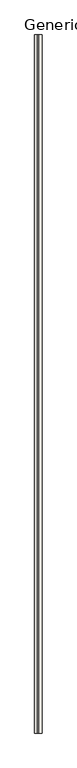
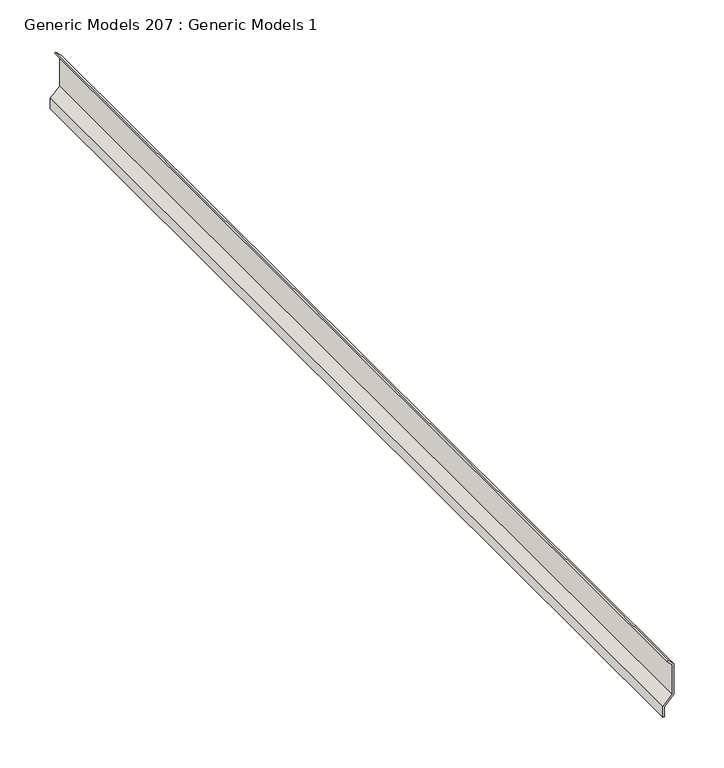
"""IFC4 building model written with IfcOpenShell, lengths in millimetres: wall geometry, Generic Models 207 : Generic Models 1."""

from ifc_helpers import new_model, si_unit, frame, origin, place, context, project, spatial, polyline, outline, extrude, source, transform, mapped, element, save


def generic_models_207_generic_models_1_57b87b31(model_context):
    return source(origin(), model_context, "Body", "SweptSolid", [
        extrude(outline(polyline([(2346.088866, 137639.6865561), (2333.388866, 137639.6865561), (2333.388866, 137641.2740561), (2345.431302, 137641.2740561), (2356.543802, 137652.3865561), (2393.713866, 137652.3865561), (2400.063866, 137646.0365561), (2398.941334, 137644.9140241), (2393.056302, 137650.7990561), (2357.201366, 137650.7990561), (2346.088866, 137639.6865561)])), frame((0.0, 0.0, 0.0), z_axis=(0.0, 1.0, 0.0), x_axis=(0.0, 0.0, 1.0)), (0.0, 0.0, 1.0), 1219.2),
    ])


if __name__ == "__main__":
    model = new_model("IFC4")
    model_context = context("Model", 3, world=origin())
    ifc_project = project(units=[si_unit("LENGTHUNIT", "METRE", prefix="MILLI")], contexts=[model_context])
    site = spatial("IfcSite", under=ifc_project)
    building = spatial("IfcBuilding", under=site)
    placement = place(None, origin())
    generic_models_207_generic_models_1_shape = generic_models_207_generic_models_1_57b87b31(model_context)
    element("IfcWall", 1, ObjectType="Generic Models 207 : Generic Models 1", at=placement, inside=building, context=model_context, shape_type="MappedRepresentation", body=[
        mapped(generic_models_207_generic_models_1_shape, transform((0.0, 0.0, 0.0), x_axis=(1.0, 0.0, 0.0), y_axis=(0.0, 1.0, 0.0), z_axis=(0.0, 0.0, 1.0))),
    ])
    save(model, "model.ifc")

# Revit data of these elements
# Element 1 (IfcWall, "Generic Models 207 : Generic Models 1")
#   Materials on its faces: "RESILIENT CHANNEL - 25 GA. FURRING CHANNELS INSTALLED HORIZONTALLY SPACED 24 IN. OC"
# Materials
#   "RESILIENT CHANNEL - 25 GA. FURRING CHANNELS INSTALLED HORIZONTALLY SPACED 24 IN. OC": class "Unassigned", colour RGB 210 209 208, transparency 0, Keynote = "M05121300.02", Cost = 0
